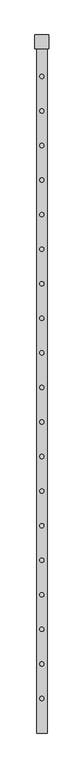
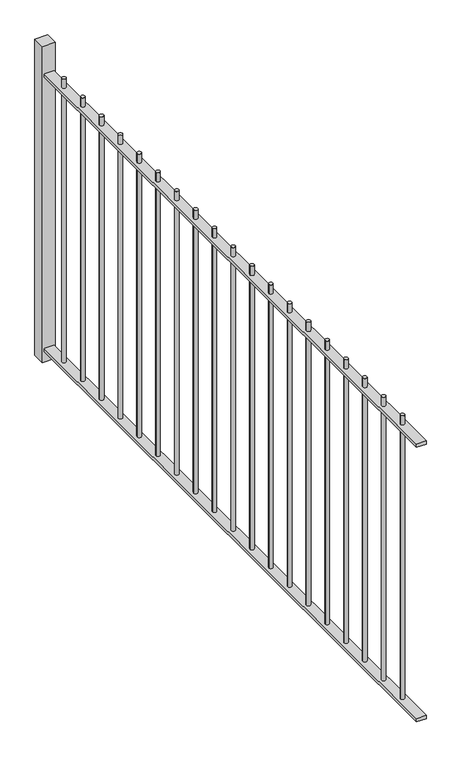
"""IFC4 building model written with IfcOpenShell, lengths in millimetres: railing geometry."""

from ifc_helpers import new_model, si_unit, point, frame, frame_2d, origin, place, context, project, spatial, polyline, circle_curve, trimmed, segment, composite_curve, outline, extrude, source, transform, mapped, element, save


def railing_d68bbb68(model_context):
    return source(origin(), model_context, "Body", "SweptSolid", [
        extrude(outline(polyline([(-6549.419961, -8771.1119119), (-6489.419961, -8771.1119119), (-6489.419961, -12771.1119119), (-6549.419961, -12771.1119119), (-6549.419961, -8771.1119119)])), frame((0.0, 0.0, -30.0), z_axis=(0.0, 0.0, 1.0), x_axis=(1.0, 0.0, 0.0)), (0.0, 0.0, 1.0), 20.0),
        extrude(outline(polyline([(-6549.419961, -8771.1119119), (-6489.419961, -8771.1119119), (-6489.419961, -12771.1119119), (-6549.419961, -12771.1119119), (-6549.419961, -8771.1119119)])), frame((0.0, 0.0, 1750.0), z_axis=(0.0, 0.0, 1.0), x_axis=(1.0, 0.0, 0.0)), (0.0, 0.0, 1.0), 20.0),
        extrude(outline(composite_curve([segment(trimmed(circle_curve(frame_2d((-6519.419961, -12571.1119119)), 12.5), [point((-6531.919961, -12571.1119119))], [point((-6506.919961, -12571.1119119))], False, "CARTESIAN"), True, "CONTINUOUS"), segment(trimmed(circle_curve(frame_2d((-6519.419961, -12571.1119119)), 12.5), [point((-6506.919961, -12571.1119119))], [point((-6531.919961, -12571.1119119))], False, "CARTESIAN"), True, "CONTINUOUS")], self_intersect=False)), frame((0.0, 0.0, -10.0), z_axis=(0.0, 0.0, 1.0), x_axis=(1.0, 0.0, 0.0)), (0.0, 0.0, 1.0), 1840.0),
        extrude(outline(composite_curve([segment(trimmed(circle_curve(frame_2d((-6519.419961, -12371.1119119)), 12.5), [point((-6531.919961, -12371.1119119))], [point((-6506.919961, -12371.1119119))], False, "CARTESIAN"), True, "CONTINUOUS"), segment(trimmed(circle_curve(frame_2d((-6519.419961, -12371.1119119)), 12.5), [point((-6506.919961, -12371.1119119))], [point((-6531.919961, -12371.1119119))], False, "CARTESIAN"), True, "CONTINUOUS")], self_intersect=False)), frame((0.0, 0.0, -10.0), z_axis=(0.0, 0.0, 1.0), x_axis=(1.0, 0.0, 0.0)), (0.0, 0.0, 1.0), 1840.0),
        extrude(outline(composite_curve([segment(trimmed(circle_curve(frame_2d((-6519.419961, -12171.1119119)), 12.5), [point((-6531.919961, -12171.1119119))], [point((-6506.919961, -12171.1119119))], False, "CARTESIAN"), True, "CONTINUOUS"), segment(trimmed(circle_curve(frame_2d((-6519.419961, -12171.1119119)), 12.5), [point((-6506.919961, -12171.1119119))], [point((-6531.919961, -12171.1119119))], False, "CARTESIAN"), True, "CONTINUOUS")], self_intersect=False)), frame((0.0, 0.0, -10.0), z_axis=(0.0, 0.0, 1.0), x_axis=(1.0, 0.0, 0.0)), (0.0, 0.0, 1.0), 1840.0),
        extrude(outline(composite_curve([segment(trimmed(circle_curve(frame_2d((-6519.419961, -11971.1119119)), 12.5), [point((-6531.919961, -11971.1119119))], [point((-6506.919961, -11971.1119119))], False, "CARTESIAN"), True, "CONTINUOUS"), segment(trimmed(circle_curve(frame_2d((-6519.419961, -11971.1119119)), 12.5), [point((-6506.919961, -11971.1119119))], [point((-6531.919961, -11971.1119119))], False, "CARTESIAN"), True, "CONTINUOUS")], self_intersect=False)), frame((0.0, 0.0, -10.0), z_axis=(0.0, 0.0, 1.0), x_axis=(1.0, 0.0, 0.0)), (0.0, 0.0, 1.0), 1840.0),
        extrude(outline(composite_curve([segment(trimmed(circle_curve(frame_2d((-6519.419961, -11771.1119119)), 12.5), [point((-6531.919961, -11771.1119119))], [point((-6506.919961, -11771.1119119))], False, "CARTESIAN"), True, "CONTINUOUS"), segment(trimmed(circle_curve(frame_2d((-6519.419961, -11771.1119119)), 12.5), [point((-6506.919961, -11771.1119119))], [point((-6531.919961, -11771.1119119))], False, "CARTESIAN"), True, "CONTINUOUS")], self_intersect=False)), frame((0.0, 0.0, -10.0), z_axis=(0.0, 0.0, 1.0), x_axis=(1.0, 0.0, 0.0)), (0.0, 0.0, 1.0), 1840.0),
        extrude(outline(composite_curve([segment(trimmed(circle_curve(frame_2d((-6519.419961, -11571.1119119)), 12.5), [point((-6531.919961, -11571.1119119))], [point((-6506.919961, -11571.1119119))], False, "CARTESIAN"), True, "CONTINUOUS"), segment(trimmed(circle_curve(frame_2d((-6519.419961, -11571.1119119)), 12.5), [point((-6506.919961, -11571.1119119))], [point((-6531.919961, -11571.1119119))], False, "CARTESIAN"), True, "CONTINUOUS")], self_intersect=False)), frame((0.0, 0.0, -10.0), z_axis=(0.0, 0.0, 1.0), x_axis=(1.0, 0.0, 0.0)), (0.0, 0.0, 1.0), 1840.0),
        extrude(outline(composite_curve([segment(trimmed(circle_curve(frame_2d((-6519.419961, -11371.1119119)), 12.5), [point((-6531.919961, -11371.1119119))], [point((-6506.919961, -11371.1119119))], False, "CARTESIAN"), True, "CONTINUOUS"), segment(trimmed(circle_curve(frame_2d((-6519.419961, -11371.1119119)), 12.5), [point((-6506.919961, -11371.1119119))], [point((-6531.919961, -11371.1119119))], False, "CARTESIAN"), True, "CONTINUOUS")], self_intersect=False)), frame((0.0, 0.0, -10.0), z_axis=(0.0, 0.0, 1.0), x_axis=(1.0, 0.0, 0.0)), (0.0, 0.0, 1.0), 1840.0),
        extrude(outline(composite_curve([segment(trimmed(circle_curve(frame_2d((-6519.419961, -11171.1119119)), 12.5), [point((-6531.919961, -11171.1119119))], [point((-6506.919961, -11171.1119119))], False, "CARTESIAN"), True, "CONTINUOUS"), segment(trimmed(circle_curve(frame_2d((-6519.419961, -11171.1119119)), 12.5), [point((-6506.919961, -11171.1119119))], [point((-6531.919961, -11171.1119119))], False, "CARTESIAN"), True, "CONTINUOUS")], self_intersect=False)), frame((0.0, 0.0, -10.0), z_axis=(0.0, 0.0, 1.0), x_axis=(1.0, 0.0, 0.0)), (0.0, 0.0, 1.0), 1840.0),
        extrude(outline(composite_curve([segment(trimmed(circle_curve(frame_2d((-6519.419961, -10971.1119119)), 12.5), [point((-6531.919961, -10971.1119119))], [point((-6506.919961, -10971.1119119))], False, "CARTESIAN"), True, "CONTINUOUS"), segment(trimmed(circle_curve(frame_2d((-6519.419961, -10971.1119119)), 12.5), [point((-6506.919961, -10971.1119119))], [point((-6531.919961, -10971.1119119))], False, "CARTESIAN"), True, "CONTINUOUS")], self_intersect=False)), frame((0.0, 0.0, -10.0), z_axis=(0.0, 0.0, 1.0), x_axis=(1.0, 0.0, 0.0)), (0.0, 0.0, 1.0), 1840.0),
        extrude(outline(composite_curve([segment(trimmed(circle_curve(frame_2d((-6519.419961, -10771.1119119)), 12.5), [point((-6531.919961, -10771.1119119))], [point((-6506.919961, -10771.1119119))], False, "CARTESIAN"), True, "CONTINUOUS"), segment(trimmed(circle_curve(frame_2d((-6519.419961, -10771.1119119)), 12.5), [point((-6506.919961, -10771.1119119))], [point((-6531.919961, -10771.1119119))], False, "CARTESIAN"), True, "CONTINUOUS")], self_intersect=False)), frame((0.0, 0.0, -10.0), z_axis=(0.0, 0.0, 1.0), x_axis=(1.0, 0.0, 0.0)), (0.0, 0.0, 1.0), 1840.0),
        extrude(outline(composite_curve([segment(trimmed(circle_curve(frame_2d((-6519.419961, -10571.1119119)), 12.5), [point((-6531.919961, -10571.1119119))], [point((-6506.919961, -10571.1119119))], False, "CARTESIAN"), True, "CONTINUOUS"), segment(trimmed(circle_curve(frame_2d((-6519.419961, -10571.1119119)), 12.5), [point((-6506.919961, -10571.1119119))], [point((-6531.919961, -10571.1119119))], False, "CARTESIAN"), True, "CONTINUOUS")], self_intersect=False)), frame((0.0, 0.0, -10.0), z_axis=(0.0, 0.0, 1.0), x_axis=(1.0, 0.0, 0.0)), (0.0, 0.0, 1.0), 1840.0),
        extrude(outline(composite_curve([segment(trimmed(circle_curve(frame_2d((-6519.419961, -10371.1119119)), 12.5), [point((-6531.919961, -10371.1119119))], [point((-6506.919961, -10371.1119119))], False, "CARTESIAN"), True, "CONTINUOUS"), segment(trimmed(circle_curve(frame_2d((-6519.419961, -10371.1119119)), 12.5), [point((-6506.919961, -10371.1119119))], [point((-6531.919961, -10371.1119119))], False, "CARTESIAN"), True, "CONTINUOUS")], self_intersect=False)), frame((0.0, 0.0, -10.0), z_axis=(0.0, 0.0, 1.0), x_axis=(1.0, 0.0, 0.0)), (0.0, 0.0, 1.0), 1840.0),
        extrude(outline(composite_curve([segment(trimmed(circle_curve(frame_2d((-6519.419961, -10171.1119119)), 12.5), [point((-6531.919961, -10171.1119119))], [point((-6506.919961, -10171.1119119))], False, "CARTESIAN"), True, "CONTINUOUS"), segment(trimmed(circle_curve(frame_2d((-6519.419961, -10171.1119119)), 12.5), [point((-6506.919961, -10171.1119119))], [point((-6531.919961, -10171.1119119))], False, "CARTESIAN"), True, "CONTINUOUS")], self_intersect=False)), frame((0.0, 0.0, -10.0), z_axis=(0.0, 0.0, 1.0), x_axis=(1.0, 0.0, 0.0)), (0.0, 0.0, 1.0), 1840.0),
        extrude(outline(composite_curve([segment(trimmed(circle_curve(frame_2d((-6519.419961, -9971.1119119)), 12.5), [point((-6531.919961, -9971.1119119))], [point((-6506.919961, -9971.1119119))], False, "CARTESIAN"), True, "CONTINUOUS"), segment(trimmed(circle_curve(frame_2d((-6519.419961, -9971.1119119)), 12.5), [point((-6506.919961, -9971.1119119))], [point((-6531.919961, -9971.1119119))], False, "CARTESIAN"), True, "CONTINUOUS")], self_intersect=False)), frame((0.0, 0.0, -10.0), z_axis=(0.0, 0.0, 1.0), x_axis=(1.0, 0.0, 0.0)), (0.0, 0.0, 1.0), 1840.0),
        extrude(outline(composite_curve([segment(trimmed(circle_curve(frame_2d((-6519.419961, -9771.1119119)), 12.5), [point((-6531.919961, -9771.1119119))], [point((-6506.919961, -9771.1119119))], False, "CARTESIAN"), True, "CONTINUOUS"), segment(trimmed(circle_curve(frame_2d((-6519.419961, -9771.1119119)), 12.5), [point((-6506.919961, -9771.1119119))], [point((-6531.919961, -9771.1119119))], False, "CARTESIAN"), True, "CONTINUOUS")], self_intersect=False)), frame((0.0, 0.0, -10.0), z_axis=(0.0, 0.0, 1.0), x_axis=(1.0, 0.0, 0.0)), (0.0, 0.0, 1.0), 1840.0),
        extrude(outline(composite_curve([segment(trimmed(circle_curve(frame_2d((-6519.419961, -9571.1119119)), 12.5), [point((-6531.919961, -9571.1119119))], [point((-6506.919961, -9571.1119119))], False, "CARTESIAN"), True, "CONTINUOUS"), segment(trimmed(circle_curve(frame_2d((-6519.419961, -9571.1119119)), 12.5), [point((-6506.919961, -9571.1119119))], [point((-6531.919961, -9571.1119119))], False, "CARTESIAN"), True, "CONTINUOUS")], self_intersect=False)), frame((0.0, 0.0, -10.0), z_axis=(0.0, 0.0, 1.0), x_axis=(1.0, 0.0, 0.0)), (0.0, 0.0, 1.0), 1840.0),
        extrude(outline(composite_curve([segment(trimmed(circle_curve(frame_2d((-6519.419961, -9371.1119119)), 12.5), [point((-6531.919961, -9371.1119119))], [point((-6506.919961, -9371.1119119))], False, "CARTESIAN"), True, "CONTINUOUS"), segment(trimmed(circle_curve(frame_2d((-6519.419961, -9371.1119119)), 12.5), [point((-6506.919961, -9371.1119119))], [point((-6531.919961, -9371.1119119))], False, "CARTESIAN"), True, "CONTINUOUS")], self_intersect=False)), frame((0.0, 0.0, -10.0), z_axis=(0.0, 0.0, 1.0), x_axis=(1.0, 0.0, 0.0)), (0.0, 0.0, 1.0), 1840.0),
        extrude(outline(composite_curve([segment(trimmed(circle_curve(frame_2d((-6519.419961, -9171.1119119)), 12.5), [point((-6531.919961, -9171.1119119))], [point((-6506.919961, -9171.1119119))], False, "CARTESIAN"), True, "CONTINUOUS"), segment(trimmed(circle_curve(frame_2d((-6519.419961, -9171.1119119)), 12.5), [point((-6506.919961, -9171.1119119))], [point((-6531.919961, -9171.1119119))], False, "CARTESIAN"), True, "CONTINUOUS")], self_intersect=False)), frame((0.0, 0.0, -10.0), z_axis=(0.0, 0.0, 1.0), x_axis=(1.0, 0.0, 0.0)), (0.0, 0.0, 1.0), 1840.0),
        extrude(outline(composite_curve([segment(trimmed(circle_curve(frame_2d((-6519.419961, -8971.1119119)), 12.5), [point((-6531.919961, -8971.1119119))], [point((-6506.919961, -8971.1119119))], False, "CARTESIAN"), True, "CONTINUOUS"), segment(trimmed(circle_curve(frame_2d((-6519.419961, -8971.1119119)), 12.5), [point((-6506.919961, -8971.1119119))], [point((-6531.919961, -8971.1119119))], False, "CARTESIAN"), True, "CONTINUOUS")], self_intersect=False)), frame((0.0, 0.0, -10.0), z_axis=(0.0, 0.0, 1.0), x_axis=(1.0, 0.0, 0.0)), (0.0, 0.0, 1.0), 1840.0),
        extrude(outline(polyline([(-6479.419961, -8731.1119119), (-6479.419961, -8811.1119119), (-6559.419961, -8811.1119119), (-6559.419961, -8731.1119119), (-6479.419961, -8731.1119119)])), frame((0.0, 0.0, -100.0), z_axis=(0.0, 0.0, 1.0), x_axis=(1.0, 0.0, 0.0)), (0.0, 0.0, 1.0), 2050.0),
    ])


if __name__ == "__main__":
    model = new_model("IFC4")
    model_context = context("Model", 3, world=origin())
    ifc_project = project(units=[si_unit("LENGTHUNIT", "METRE", prefix="MILLI")], contexts=[model_context])
    site = spatial("IfcSite", under=ifc_project)
    building = spatial("IfcBuilding", under=site)
    placement = place(None, origin())
    railing_shape = railing_d68bbb68(model_context)
    element("IfcRailing", 1, at=placement, inside=building, context=model_context, shape_type="MappedRepresentation", body=[
        mapped(railing_shape, transform((0.0, 0.0, 0.0), x_axis=(1.0, 0.0, 0.0), y_axis=(0.0, 1.0, 0.0), z_axis=(0.0, 0.0, 1.0))),
    ])
    save(model, "model.ifc")

# Revit data of these elements
# Element 1 (IfcRailing)
#   Materials on its faces: "NLRS_h2_staal_generiek zwart_gen_rsf", "NLRS_h2_staal_gen_rsf"
# Materials
#   "NLRS_h2_staal_generiek zwart_gen_rsf": class "Metal", colour RGB 189 187 185, transparency 0, Manufacturer = "RevitGG", URL = "www.revitgg.nl", Description = "Staal, generiek materiaal", Cost = 0
#   "NLRS_h2_staal_gen_rsf": class "H - Metaal", colour RGB 189 187 185, transparency 0, Keynote = "h2", Model = "generiek", Manufacturer = "Revit Standards Foundation", URL = "www.revitstandards.org", Description = "staal", Cost = 0
